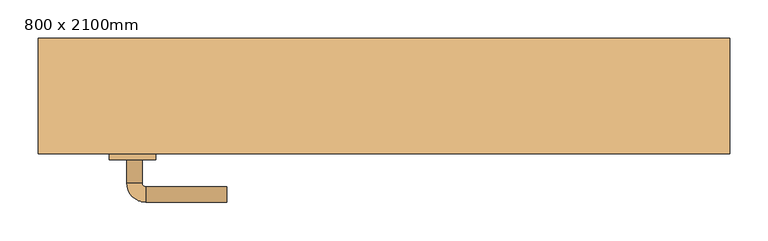
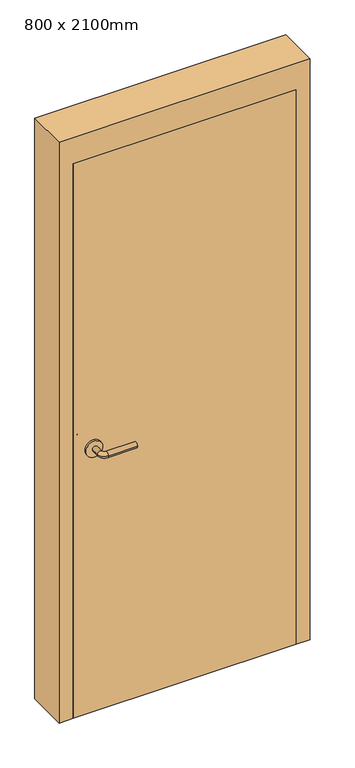
"""IFC4 building model written with IfcOpenShell, lengths in millimetres: door geometry, M_Puerta-De_paso-Simple-Paneles_planos : 800 x 2100mm."""

from ifc_helpers import new_model, si_unit, point, frame, frame_2d, origin, origin_with_axes, place, context, project, spatial, polyline, circle_curve, ellipse_curve, trimmed, segment, composite_curve, outline, extrude, faceted_brep, source, transform, mapped, element, save
from ifc_brep_helpers import plane_surface, cylinder_surface, revolved_surface, advanced_brep


def door_800_x_2100mm_8b307582(model_context):
    return source(origin(), model_context, "Body", "SolidModel", [
        advanced_brep(
        [(-334.990625, -3.35, 1000.0), (-314.990625, -3.35, 1000.0), (-334.990625, 26.65, 1000.0), (-314.990625, 26.65, 1000.0), (-309.990625, 31.65, 1000.0), (-309.990625, 51.65, 1000.0), (-204.990625, 51.65, 1000.0), (-204.990625, 31.65, 1000.0)],
        [
            (0, 1, circle_curve(frame((-324.990625, -3.35, 1000.0), z_axis=(0.0, -1.0, 0.0), x_axis=(1.0, 0.0, 0.0)), 10.0)),
            (1, 0, circle_curve(frame((-324.990625, -3.35, 1000.0), z_axis=(0.0, -1.0, 0.0), x_axis=(1.0, 0.0, 0.0)), 10.0)),
            (0, 2),
            (2, 3, circle_curve(frame((-324.990625, 26.65, 1000.0), z_axis=(0.0, -1.0, 0.0), x_axis=(1.0, 0.0, 0.0)), 10.0)),
            (3, 1),
            (3, 2, circle_curve(frame((-324.990625, 26.65, 1000.0), z_axis=(0.0, -1.0, 0.0), x_axis=(1.0, 0.0, 0.0)), 10.0)),
            (4, 3, circle_curve(frame((-309.990625, 26.65, 1000.0), z_axis=(0.0, 0.0, 1.0), x_axis=(-1.0, 0.0, 0.0)), 5.0)),
            (2, 5, circle_curve(frame((-309.990625, 26.65, 1000.0), z_axis=(0.0, 0.0, -1.0), x_axis=(-1.0, 0.0, 0.0)), 25.0)),
            (5, 4, circle_curve(frame((-309.990625, 41.65, 1000.0), z_axis=(-1.0, 0.0, 0.0), x_axis=(0.0, -1.0, 0.0)), 10.0)),
            (4, 5, circle_curve(frame((-309.990625, 41.65, 1000.0), z_axis=(-1.0, 0.0, 0.0), x_axis=(0.0, -1.0, 0.0)), 10.0)),
            (6, 7, circle_curve(frame((-204.990625, 41.65, 1000.0), z_axis=(1.0, 0.0, 0.0), x_axis=(0.0, -1.0, 0.0)), 10.0)),
            (7, 6, circle_curve(frame((-204.990625, 41.65, 1000.0), z_axis=(1.0, 0.0, 0.0), x_axis=(0.0, -1.0, 0.0)), 10.0)),
            (5, 6),
            (7, 4),
        ],
        [
            plane_surface(frame((-324.990625, -3.35, 1000.0), z_axis=(0.0, -1.0, 0.0), x_axis=(0.0, 0.0, 1.0))),
            cylinder_surface(frame((-324.990625, -3.35, 1000.0), z_axis=(0.0, -1.0, 0.0), x_axis=(1.0, 0.0, 0.0)), 10.0),
            revolved_surface(trimmed(ellipse_curve(frame((-324.990625, 26.65, 1000.0), z_axis=(0.0, -1.0, 0.0), x_axis=(1.0, 0.0, 0.0)), 10.0, 10.0), [point((-334.990625, 26.65, 1000.0))], [point((-314.990625, 26.65, 1000.0))], True, "CARTESIAN"), (-309.990625, 26.65, 1000.0), (0.0, 0.0, -1.0)),
            revolved_surface(trimmed(ellipse_curve(frame((-324.990625, 26.65, 1000.0), z_axis=(0.0, -1.0, 0.0), x_axis=(1.0, 0.0, 0.0)), 10.0, 10.0), [point((-314.990625, 26.65, 1000.0))], [point((-334.990625, 26.65, 1000.0))], True, "CARTESIAN"), (-309.990625, 26.65, 1000.0), (0.0, 0.0, -1.0)),
            plane_surface(frame((-204.990625, 41.65, 1000.0), z_axis=(1.0, 0.0, 0.0), x_axis=(0.0, 0.0, 1.0))),
            cylinder_surface(frame((-309.990625, 41.65, 1000.0), z_axis=(-1.0, 0.0, 0.0), x_axis=(0.0, -1.0, 0.0)), 10.0),
        ],
        [
            (0, [[1, 2]]),
            (1, [[-1, 3, 4, 5]]),
            (1, [[-2, -5, 6, -3]]),
            (2, [[7, -4, 8, 9]]),
            (3, [[-8, -6, -7, 10]]),
            (4, [[11, 12]]),
            (5, [[-9, 13, -12, 14]]),
            (5, [[-10, -14, -11, -13]]),
        ],
    ),
        extrude(outline(composite_curve([segment(trimmed(circle_curve(frame_2d((1000.0, -327.490625)), 30.0), [point((1000.0, -357.490625))], [point((1000.0, -297.490625))], False, "CARTESIAN"), True, "CONTINUOUS"), segment(trimmed(circle_curve(frame_2d((1000.0, -327.490625)), 30.0), [point((1000.0, -297.490625))], [point((1000.0, -357.490625))], False, "CARTESIAN"), True, "CONTINUOUS")], self_intersect=False)), frame((0.0, -11.35, 0.0), z_axis=(0.0, 1.0, 0.0), x_axis=(0.0, 0.0, 1.0)), (0.0, 0.0, 1.0), 8.0),
        advanced_brep(
        [(-334.990625, -64.35, 1000.0), (-314.990625, -64.35, 1000.0), (-314.990625, -94.35, 1000.0), (-334.990625, -94.35, 1000.0), (-309.990625, -99.35, 1000.0), (-309.990625, -119.35, 1000.0), (-204.990625, -119.35, 1000.0), (-204.990625, -99.35, 1000.0)],
        [
            (0, 1, circle_curve(frame((-324.990625, -64.35, 1000.0), z_axis=(0.0, 1.0, 0.0), x_axis=(1.0, 0.0, 0.0)), 10.0)),
            (1, 0, circle_curve(frame((-324.990625, -64.35, 1000.0), z_axis=(0.0, 1.0, 0.0), x_axis=(1.0, 0.0, 0.0)), 10.0)),
            (1, 2),
            (2, 3, circle_curve(frame((-324.990625, -94.35, 1000.0), z_axis=(0.0, 1.0, 0.0), x_axis=(1.0, 0.0, 0.0)), 10.0)),
            (3, 0),
            (3, 2, circle_curve(frame((-324.990625, -94.35, 1000.0), z_axis=(0.0, 1.0, 0.0), x_axis=(1.0, 0.0, 0.0)), 10.0)),
            (4, 5, circle_curve(frame((-309.990625, -109.35, 1000.0), z_axis=(-1.0, 0.0, 0.0), x_axis=(0.0, 1.0, 0.0)), 10.0)),
            (5, 3, circle_curve(frame((-309.990625, -94.35, 1000.0), z_axis=(0.0, 0.0, -1.0), x_axis=(-1.0, 0.0, 0.0)), 25.0)),
            (2, 4, circle_curve(frame((-309.990625, -94.35, 1000.0), z_axis=(0.0, 0.0, 1.0), x_axis=(-1.0, 0.0, 0.0)), 5.0)),
            (5, 4, circle_curve(frame((-309.990625, -109.35, 1000.0), z_axis=(-1.0, 0.0, 0.0), x_axis=(0.0, 1.0, 0.0)), 10.0)),
            (6, 7, circle_curve(frame((-204.990625, -109.35, 1000.0), z_axis=(1.0, 0.0, 0.0), x_axis=(0.0, 1.0, 0.0)), 10.0)),
            (7, 6, circle_curve(frame((-204.990625, -109.35, 1000.0), z_axis=(1.0, 0.0, 0.0), x_axis=(0.0, 1.0, 0.0)), 10.0)),
            (4, 7),
            (6, 5),
        ],
        [
            plane_surface(frame((-324.990625, -64.35, 1000.0), z_axis=(0.0, 1.0, 0.0), x_axis=(0.0, 0.0, 1.0))),
            cylinder_surface(frame((-324.990625, -64.35, 1000.0), z_axis=(0.0, 1.0, 0.0), x_axis=(1.0, 0.0, 0.0)), 10.0),
            revolved_surface(trimmed(ellipse_curve(frame((-324.990625, -94.35, 1000.0), z_axis=(0.0, -1.0, 0.0), x_axis=(1.0, 0.0, 0.0)), 10.0, 10.0), [point((-334.990625, -94.35, 1000.0))], [point((-314.990625, -94.35, 1000.0))], True, "CARTESIAN"), (-309.990625, -94.35, 1000.0), (0.0, 0.0, -1.0)),
            revolved_surface(trimmed(ellipse_curve(frame((-324.990625, -94.35, 1000.0), z_axis=(0.0, -1.0, 0.0), x_axis=(1.0, 0.0, 0.0)), 10.0, 10.0), [point((-314.990625, -94.35, 1000.0))], [point((-334.990625, -94.35, 1000.0))], True, "CARTESIAN"), (-309.990625, -94.35, 1000.0), (0.0, 0.0, -1.0)),
            plane_surface(frame((-204.990625, -109.35, 1000.0), z_axis=(1.0, 0.0, 0.0), x_axis=(0.0, 0.0, 1.0))),
            cylinder_surface(frame((-309.990625, -109.35, 1000.0), z_axis=(-1.0, 0.0, 0.0), x_axis=(0.0, 1.0, 0.0)), 10.0),
        ],
        [
            (0, [[1, 2]]),
            (1, [[3, 4, 5, -2]]),
            (1, [[-5, 6, -3, -1]]),
            (2, [[7, 8, -4, 9]]),
            (3, [[10, -9, -6, -8]]),
            (4, [[11, 12]]),
            (5, [[13, -11, 14, -7]]),
            (5, [[-14, -12, -13, -10]]),
        ],
    ),
        extrude(outline(composite_curve([segment(trimmed(circle_curve(frame_2d((1000.0, -327.490625)), 30.0), [point((1000.0, -357.490625))], [point((1000.0, -297.490625))], False, "CARTESIAN"), True, "CONTINUOUS"), segment(trimmed(circle_curve(frame_2d((1000.0, -327.490625)), 30.0), [point((1000.0, -297.490625))], [point((1000.0, -357.490625))], False, "CARTESIAN"), True, "CONTINUOUS")], self_intersect=False)), frame((0.0, -64.35, 0.0), z_axis=(0.0, 1.0, 0.0), x_axis=(0.0, 0.0, 1.0)), (0.0, 0.0, 1.0), 8.0),
        extrude(outline(polyline([(400.0, -11.35), (400.0, -56.35), (-400.0, -56.35), (-400.0, -11.35), (400.0, -11.35)])), origin_with_axes(), (0.0, 0.0, 1.0), 2100.0),
        faceted_brep([(400.0, -6.5875, 0.0), (384.125, -6.5875, 0.0), (384.125, 44.4375, 0.0), (400.0, 44.4375, 0.0), (400.0, 93.65, 0.0), (450.0, 93.65, 0.0), (450.0, -56.35, 0.0), (400.0, -56.35, 0.0), (400.0, -56.35, 2100.0), (400.0, -6.5875, 2100.0), (450.0, -56.35, 2200.0), (-450.0, -56.35, 2200.0), (-450.0, -56.35, 0.0), (-400.0, -56.35, 0.0), (-400.0, -56.35, 2100.0), (450.0, 93.65, 2200.0), (400.0, 93.65, 2100.0), (-400.0, 93.65, 2100.0), (-400.0, 93.65, 0.0), (-450.0, 93.65, 0.0), (-450.0, 93.65, 2200.0), (400.0, 44.4375, 2100.0), (384.125, 44.4375, 2084.125), (-384.125, 44.4375, 2084.125), (-384.125, 44.4375, 0.0), (-400.0, 44.4375, 0.0), (-400.0, 44.4375, 2100.0), (384.125, -6.5875, 2084.125), (-400.0, -6.5875, 2100.0), (-400.0, -6.5875, 0.0), (-384.125, -6.5875, 0.0), (-384.125, -6.5875, 2084.125)], [[[0, 1, 2, 3, 4, 5, 6, 7]], [[7, 8, 9, 0]], [[6, 10, 11, 12, 13, 14, 8, 7]], [[5, 15, 10, 6]], [[4, 16, 17, 18, 19, 20, 15, 5]], [[3, 21, 16, 4]], [[2, 22, 23, 24, 25, 26, 21, 3]], [[1, 27, 22, 2]], [[0, 9, 28, 29, 30, 31, 27, 1]], [[8, 14, 28, 9]], [[16, 21, 26, 17]], [[22, 27, 31, 23]], [[12, 19, 18, 25, 24, 30, 29, 13]], [[13, 29, 28, 14]], [[11, 20, 19, 12]], [[17, 26, 25, 18]], [[23, 31, 30, 24]], [[15, 20, 11, 10]]]),
    ])


if __name__ == "__main__":
    model = new_model("IFC4")
    model_context = context("Model", 3, world=origin())
    ifc_project = project(units=[si_unit("LENGTHUNIT", "METRE", prefix="MILLI")], contexts=[model_context])
    site = spatial("IfcSite", under=ifc_project)
    building = spatial("IfcBuilding", under=site)
    placement = place(None, origin())
    door_800_x_2100mm_shape = door_800_x_2100mm_8b307582(model_context)
    element("IfcDoor", 1, ObjectType="M_Puerta-De_paso-Simple-Paneles_planos : 800 x 2100mm", at=placement, inside=building, context=model_context, shape_type="MappedRepresentation", body=[
        mapped(door_800_x_2100mm_shape, transform((0.0, 0.0, 0.0), x_axis=(1.0, 0.0, 0.0), y_axis=(0.0, 1.0, 0.0), z_axis=(0.0, 0.0, 1.0))),
    ])
    save(model, "model.ifc")

# Revit data of these elements
# Type "M_Puerta-De_paso-Simple-Paneles_planos : 800 x 2100mm"
#   Type Mark = "47"
#   Analytic Construction = "Madera"
#   Thickness = 0.045 m
#   Thermal Resistance (R) = 0.455703 (m²·K)/W
#   Ángulo de batiente [instance default] = 90.00°
#   Altura del pasador = 1.00 m
#   Rough Width [instance default] = 0.90 m
#   Rough Height [instance default] = 2.20 m
#   Altura de hueco MF [instance default] = 0.10 m
#   Anchura de hueco MF [instance default] = 0.10 m
#   Cálculo de la incrustación [instance default] = 0.105 m
#   Incrustación de albañilería [instance default] = 0.025 m
#   Height = 2.10 m
#   Width = 0.80 m
#   Heat Transfer Coefficient (U) = 2.19465 W/(m²·K)
#   Profundidad del marco del albañilería = 0.15 m
#   Marco del albañilería [instance default] = yes
#   Function = 1
#   Marco de muro seco [instance default] = no
#   Material de panel = Madera - Abedul
#   Material de estructura = Metal - Acabado de pintura - Gris
#   Material de tirador = Aluminio 1
#   Visual Light Transmittance = 0
#   Solar Heat Gain Coefficient = 0
#   Wall Closure = (empty or 0)
# Element 1 (IfcDoor, "M_Puerta-De_paso-Simple-Paneles_planos : 800 x 2100mm")
#   Materials on its faces: "Aluminio 1", "Metal - Acabado de pintura - Gris", "Madera - Abedul"
# Materials
#   "Madera - Abedul": class "Madera", colour RGB 173 132 96, transparency 0, Cost = 0
#   "Metal - Acabado de pintura - Gris": class "Pintura", colour RGB 178 178 178, transparency 0, Cost = 0
#   "Aluminio 1": class "Metal", colour RGB 244 245 246, transparency 0, Description = "Aluminio 6061", Cost = 0
